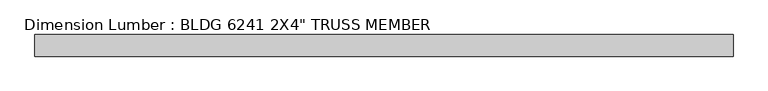
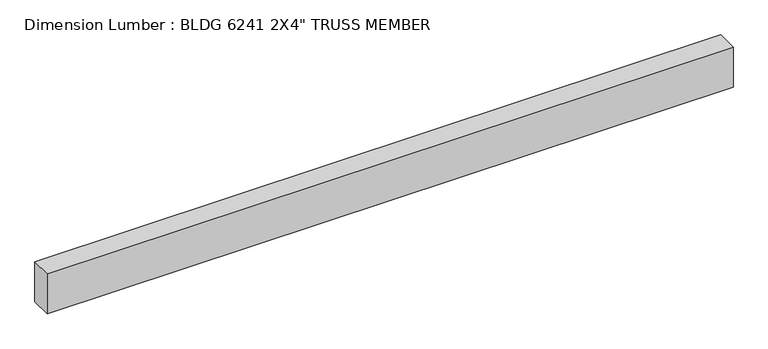
"""IFC4 building model written with IfcOpenShell, lengths in millimetres: beam geometry."""

from ifc_helpers import new_model, si_unit, frame, origin, place, context, project, spatial, polyline, outline, extrude, source, transform, mapped, element, save


def beam_16181373(model_context):
    return source(origin(), model_context, "Body", "SweptSolid", [
        extrude(outline(polyline([(819.5010489, 25.4), (819.5010489, -25.4), (-821.193698, -25.4), (-821.193698, 25.4), (819.5010489, 25.4)])), frame((0.0, 0.0, -50.8), z_axis=(0.0, 0.0, 1.0), x_axis=(1.0, 0.0, 0.0)), (0.0, 0.0, 1.0), 101.6),
    ])


if __name__ == "__main__":
    model = new_model("IFC4")
    model_context = context("Model", 3, world=origin())
    ifc_project = project(units=[si_unit("LENGTHUNIT", "METRE", prefix="MILLI")], contexts=[model_context])
    site = spatial("IfcSite", under=ifc_project)
    building = spatial("IfcBuilding", under=site)
    placement = place(None, origin())
    beam_shape = beam_16181373(model_context)
    element("IfcBeam", 1, ObjectType="Dimension Lumber : BLDG 6241 2X4\" TRUSS MEMBER", at=placement, inside=building, context=model_context, shape_type="MappedRepresentation", body=[
        mapped(beam_shape, transform((0.0, 0.0, 0.0), x_axis=(1.0, 0.0, 0.0), y_axis=(0.0, 1.0, 0.0), z_axis=(0.0, 0.0, 1.0))),
    ])
    save(model, "model.ifc")

# Revit data of these elements
# Type "Dimension Lumber : BLDG 6241 2X4\" TRUSS MEMBER"
#   Assembly Code = "B10"
#   A = 0.273472 SF
#   Length [instance default] = 5' - 0"
#   b = 0' - 2"
#   d = 0' - 4"
#   Structural Material [instance default] = Softwood, Lumber
# Element 1 (IfcBeam, "Dimension Lumber : BLDG 6241 2X4\" TRUSS MEMBER")
#   Materials on its faces: "Softwood, Lumber"
# Materials
#   "Softwood, Lumber": class "Wood", colour RGB 223 192 134, transparency 0, Description = "Pinus Echinata", Cost = 0
